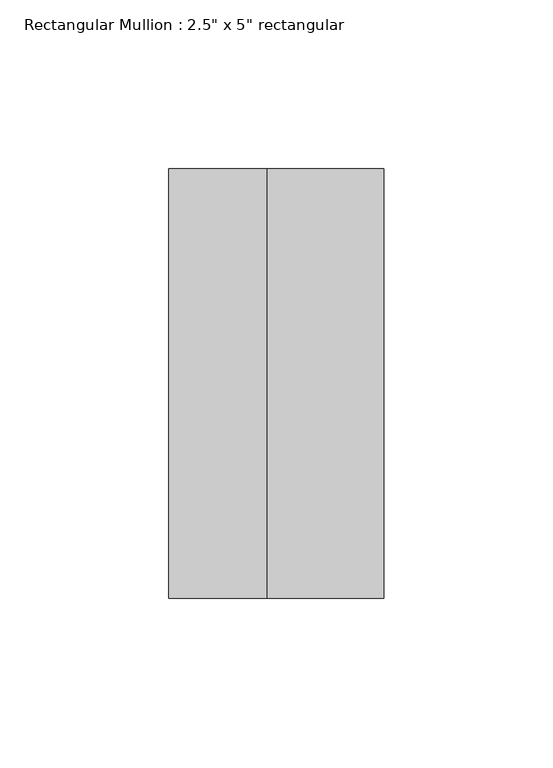
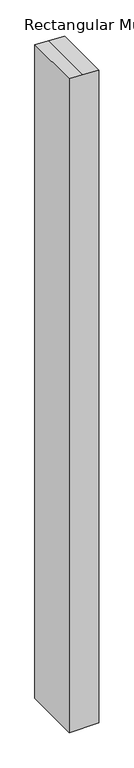
"""IFC4 building model written with IfcOpenShell, lengths in millimetres: member geometry."""

from ifc_helpers import new_model, si_unit, frame, origin, place, context, project, spatial, polyline, outline, extrude, source, transform, mapped, element, save


def member_4e2f7fd9(model_context):
    return source(origin(), model_context, "Body", "SweptSolid", [
        extrude(outline(polyline([(-64.8775557, 31.75), (-63.4449853, -2.6426951), (-62.232569, -31.75), (-1539.2879787, -31.75), (-1539.2879787, 31.75), (-64.8775557, 31.75)])), frame((0.0, -63.5, 0.0), z_axis=(0.0, 1.0, 0.0), x_axis=(0.0, 0.0, 1.0)), (0.0, 0.0, 1.0), 127.0),
    ])


if __name__ == "__main__":
    model = new_model("IFC4")
    model_context = context("Model", 3, world=origin())
    ifc_project = project(units=[si_unit("LENGTHUNIT", "METRE", prefix="MILLI")], contexts=[model_context])
    site = spatial("IfcSite", under=ifc_project)
    building = spatial("IfcBuilding", under=site)
    placement = place(None, origin())
    member_shape = member_4e2f7fd9(model_context)
    element("IfcMember", 1, ObjectType="Rectangular Mullion : 2.5\" x 5\" rectangular", at=placement, inside=building, context=model_context, shape_type="MappedRepresentation", body=[
        mapped(member_shape, transform((0.0, 0.0, 0.0), x_axis=(1.0, 0.0, 0.0), y_axis=(0.0, 1.0, 0.0), z_axis=(0.0, 0.0, 1.0))),
    ])
    save(model, "model.ifc")

# Revit data of these elements
# Type "Rectangular Mullion : 2.5\" x 5\" rectangular"
#   built-in parameter 1007304 = 0.416667 (stored number, unit not read)
#   built-in parameter 1007301 = 0.104167 (stored number, unit not read)
#   built-in parameter 1007300 = 0.104167 (stored number, unit not read)
# Element 1 (IfcMember, "Rectangular Mullion : 2.5\" x 5\" rectangular")
#   Materials on its faces: "Aluminum"
# Materials
#   "Aluminum": class "Metal", colour RGB 247 247 247, transparency 0, Description = "Aluminum 6061", Cost = 0
